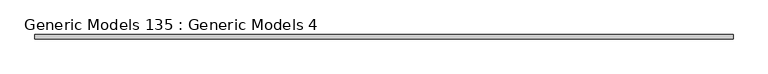
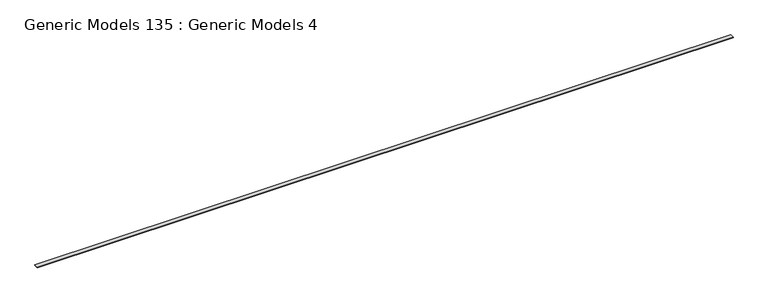
"""IFC4 building model written with IfcOpenShell, lengths in millimetres: proxy geometry, Generic Models 135 : Generic Models 4."""

from ifc_helpers import new_model, si_unit, frame, origin, place, context, project, spatial, polyline, outline, extrude, source, transform, mapped, element, save


def generic_models_135_generic_models_4_fa114a06(model_context):
    return source(origin(), model_context, "Body", "SweptSolid", [
        extrude(outline(polyline([(21700.7658099, 13370.5639146), (21700.7658099, 13282.8745053), (7781.5658099, 13282.8745053), (7781.5658099, 13370.5639146), (21700.7658099, 13370.5639146)])), frame((0.0, 0.0, 129263.3128468), z_axis=(0.0, 0.0, 1.0), x_axis=(1.0, 0.0, 0.0)), (0.0, 0.0, 1.0), 9.525),
    ])


if __name__ == "__main__":
    model = new_model("IFC4")
    model_context = context("Model", 3, world=origin())
    ifc_project = project(units=[si_unit("LENGTHUNIT", "METRE", prefix="MILLI")], contexts=[model_context])
    site = spatial("IfcSite", under=ifc_project)
    building = spatial("IfcBuilding", under=site)
    placement = place(None, origin())
    generic_models_135_generic_models_4_shape = generic_models_135_generic_models_4_fa114a06(model_context)
    element("IfcBuildingElementProxy", 1, Name="Generic Models 135 : Generic Models 4", ObjectType="Generic Models 135 : Generic Models 4", at=placement, inside=building, context=model_context, shape_type="MappedRepresentation", body=[
        mapped(generic_models_135_generic_models_4_shape, transform((0.0, 0.0, 0.0), x_axis=(1.0, 0.0, 0.0), y_axis=(0.0, 1.0, 0.0), z_axis=(0.0, 0.0, 1.0))),
    ])
    save(model, "model.ifc")

# Revit data of these elements
# Element 1 (IfcBuildingElementProxy, "Generic Models 135 : Generic Models 4")
#   Materials on its faces: "_BLOCKING AS REQUIRED"
# Materials
#   "_BLOCKING AS REQUIRED": class "Generic", colour RGB 177 130 114, transparency 0, Cost = 0
